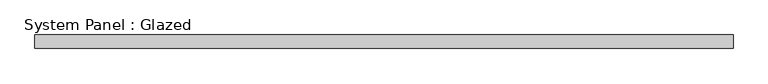
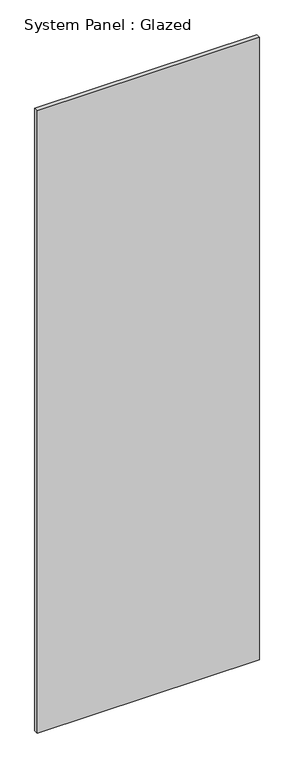
"""IFC4 building model written with IfcOpenShell, lengths in millimetres: plate geometry, System Panel : Glazed."""

from ifc_helpers import new_model, si_unit, origin, origin_with_axes, place, context, project, spatial, polyline, outline, extrude, source, transform, mapped, element, save


def system_panel_glazed_f91df05e(model_context):
    return source(origin(), model_context, "Body", "SweptSolid", [
        extrude(outline(polyline([(660.033654, 19.05), (-660.033654, 19.05), (-660.033654, 44.45), (660.033654, 44.45), (660.033654, 19.05)])), origin_with_axes(), (0.0, 0.0, 1.0), 3908.2835741),
    ])


if __name__ == "__main__":
    model = new_model("IFC4")
    model_context = context("Model", 3, world=origin())
    ifc_project = project(units=[si_unit("LENGTHUNIT", "METRE", prefix="MILLI")], contexts=[model_context])
    site = spatial("IfcSite", under=ifc_project)
    building = spatial("IfcBuilding", under=site)
    placement = place(None, origin())
    system_panel_glazed_shape = system_panel_glazed_f91df05e(model_context)
    element("IfcPlate", 1, ObjectType="System Panel : Glazed", at=placement, inside=building, context=model_context, shape_type="MappedRepresentation", body=[
        mapped(system_panel_glazed_shape, transform((0.0, 0.0, 0.0), x_axis=(1.0, 0.0, 0.0), y_axis=(0.0, 1.0, 0.0), z_axis=(0.0, 0.0, 1.0))),
    ])
    save(model, "model.ifc")

# Revit data of these elements
# Type "System Panel : Glazed"
#   Construction Type Id = "GSP4R"
#   Analytic Construction = "1/8 in Pilkington single glazing"
#   Visual Light Transmittance = 0.9
#   Solar Heat Gain Coefficient = 0.86
#   Heat Transfer Coefficient (U) = 1.18115 BTU/(h·ft²·°F)
#   Define Thermal Properties by = 1
# Element 1 (IfcPlate, "System Panel : Glazed")
#   Materials on its faces: "Glass"
# Materials
#   "Glass": class "Glass", colour RGB 0 128 192, transparency 0.75, Description = "Soda Lime Glass", Cost = 0
